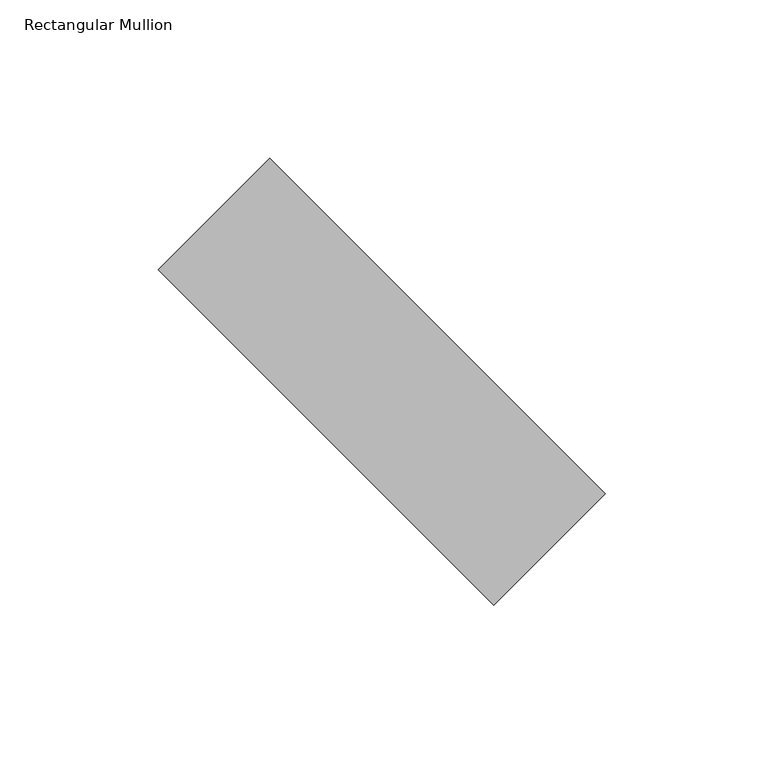
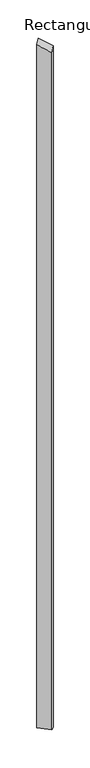
"""IFC4 building model written with IfcOpenShell, lengths in millimetres: member geometry, Rectangular Mullion : tilted mullions."""

from ifc_helpers import new_model, si_unit, origin, place, context, project, spatial, faceted_brep, source, transform, mapped, element, save


def rectangular_mullion_9c5b585c(model_context):
    return source(origin(), model_context, "Body", "Brep", [
        faceted_brep([(-35.3553391, 70.7106781, -7999.2474034), (70.7106781, -35.3553391, -7999.2474034), (35.3553391, -70.7106781, -7999.2474034), (-70.7106781, 35.3553391, -7999.2474034), (-70.7106781, 35.3553391, 10.0945584), (-35.3553391, 70.7106781, 55.1215388), (35.3553391, -70.7106781, -55.1215388), (70.7106781, -35.3553391, -10.0945584)], [[[0, 1, 2, 3]], [[4, 5, 0, 3]], [[6, 4, 3, 2]], [[7, 6, 2, 1]], [[5, 7, 1, 0]], [[5, 4, 6, 7]]]),
    ])


if __name__ == "__main__":
    model = new_model("IFC4")
    model_context = context("Model", 3, world=origin())
    ifc_project = project(units=[si_unit("LENGTHUNIT", "METRE", prefix="MILLI")], contexts=[model_context])
    site = spatial("IfcSite", under=ifc_project)
    building = spatial("IfcBuilding", under=site)
    placement = place(None, origin())
    rectangular_mullion_shape = rectangular_mullion_9c5b585c(model_context)
    element("IfcMember", 1, ObjectType="Rectangular Mullion : tilted mullions", at=placement, inside=building, context=model_context, shape_type="MappedRepresentation", body=[
        mapped(rectangular_mullion_shape, transform((0.0, 0.0, 0.0), x_axis=(1.0, 0.0, 0.0), y_axis=(0.0, 1.0, 0.0), z_axis=(0.0, 0.0, 1.0))),
    ])
    save(model, "model.ifc")

# Revit data of these elements
# Type "Rectangular Mullion : tilted mullions"
#   built-in parameter 1007304 = 0.492126 (stored number, unit not read)
#   built-in parameter 1007301 = 0.082021 (stored number, unit not read)
#   built-in parameter 1007300 = 0.082021 (stored number, unit not read)
# Element 1 (IfcMember, "Rectangular Mullion : tilted mullions")
#   Materials on its faces: "Aluminum"
# Materials
#   "Aluminum": class "Metal", colour RGB 244 244 244, transparency 0, Description = "Aluminum 6061", Cost = 0
